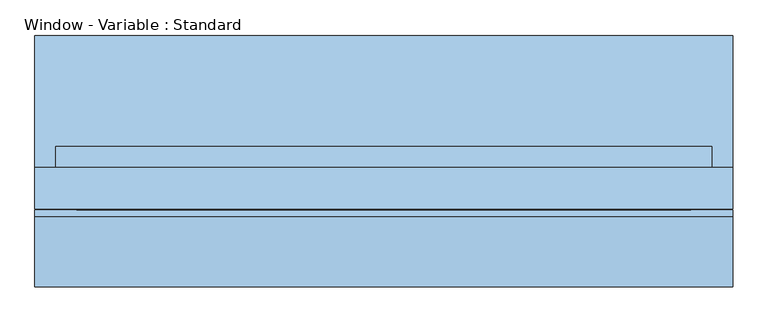
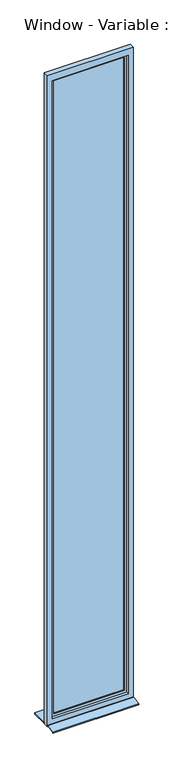
"""IFC4 building model written with IfcOpenShell, lengths in millimetres: window geometry, Window - Variable : Standard."""

from ifc_helpers import new_model, si_unit, frame, origin, place, context, project, spatial, polyline, outline, extrude, faceted_brep, source, transform, mapped, element, save


def window_variable_standard_9eb8f332(model_context):
    return source(origin(), model_context, "Body", "SolidModel", [
        extrude(outline(polyline([(9000.0, 500.0), (9000.0, -500.0), (1000.0, -500.0), (1000.0, 500.0), (9000.0, 500.0)]), holes=[polyline([(8920.0, 440.0), (1080.0, 440.0), (1080.0, -440.0), (8920.0, -440.0), (8920.0, 440.0)])]), frame((0.0, -70.0, 0.0), z_axis=(0.0, 1.0, 0.0), x_axis=(0.0, 0.0, 1.0)), (0.0, 0.0, 1.0), 60.0),
        faceted_brep([(470.0, -10.0, 8950.0), (470.0, -10.0, 1050.0), (470.0, 20.0, 1050.0), (470.0, 20.0, 8950.0), (-470.0, 20.0, 1050.0), (-470.0, 20.0, 8950.0), (410.0, 20.0, 1110.0), (410.0, 20.0, 8890.0), (-410.0, 20.0, 8890.0), (-410.0, 20.0, 1110.0), (-470.0, -10.0, 1050.0), (-470.0, -10.0, 8950.0), (440.0, -10.0, 8920.0), (440.0, -10.0, 1080.0), (-440.0, -10.0, 1080.0), (-440.0, -10.0, 8920.0), (440.0, -40.0, 8920.0), (440.0, -40.0, 1080.0), (-440.0, -40.0, 1080.0), (-440.0, -40.0, 8920.0), (410.0, -40.0, 8890.0), (410.0, -40.0, 1110.0), (-410.0, -40.0, 1110.0), (-410.0, -40.0, 8890.0)], [[[0, 1, 2, 3]], [[3, 2, 4, 5], [6, 7, 8, 9]], [[1, 10, 4, 2]], [[1, 0, 11, 10], [12, 13, 14, 15]], [[16, 17, 13, 12]], [[17, 18, 14, 13]], [[17, 16, 19, 18], [20, 21, 22, 23]], [[7, 6, 21, 20]], [[6, 9, 22, 21]], [[10, 11, 5, 4]], [[18, 19, 15, 14]], [[9, 8, 23, 22]], [[11, 0, 3, 5]], [[19, 16, 12, 15]], [[8, 7, 20, 23]]]),
        extrude(outline(polyline([(-500.0, 180.0), (500.0, 180.0), (500.0, -10.0), (-500.0, -10.0), (-500.0, 180.0)])), frame((0.0, 0.0, 1005.0), z_axis=(0.0, 0.0, 1.0), x_axis=(1.0, 0.0, 0.0)), (0.0, 0.0, 1.0), 15.0),
        extrude(outline(polyline([(-80.0221543, 1020.0), (-70.0, 1020.0), (-70.0, 1018.0), (-79.8240723, 1018.0), (-178.0, 998.3604634), (-178.0, 990.0), (-180.0, 990.0), (-180.0, 1000.0), (-80.0221543, 1020.0)])), frame((-500.0, 0.0, 0.0), z_axis=(1.0, 0.0, 0.0), x_axis=(0.0, 1.0, 0.0)), (0.0, 0.0, 1.0), 1000.0),
        extrude(outline(polyline([(410.0, 5.0), (410.0, -25.0), (-410.0, -25.0), (-410.0, 5.0), (410.0, 5.0)])), frame((0.0, 0.0, 1110.0), z_axis=(0.0, 0.0, 1.0), x_axis=(1.0, 0.0, 0.0)), (0.0, 0.0, 1.0), 7780.0),
    ])


if __name__ == "__main__":
    model = new_model("IFC4")
    model_context = context("Model", 3, world=origin())
    ifc_project = project(units=[si_unit("LENGTHUNIT", "METRE", prefix="MILLI")], contexts=[model_context])
    site = spatial("IfcSite", under=ifc_project)
    building = spatial("IfcBuilding", under=site)
    placement = place(None, origin())
    window_variable_standard_shape = window_variable_standard_9eb8f332(model_context)
    element("IfcWindow", 1, ObjectType="Window - Variable : Standard", at=placement, inside=building, context=model_context, shape_type="MappedRepresentation", body=[
        mapped(window_variable_standard_shape, transform((0.0, 0.0, 0.0), x_axis=(1.0, 0.0, 0.0), y_axis=(0.0, 1.0, 0.0), z_axis=(0.0, 0.0, 1.0))),
    ])
    save(model, "model.ifc")

# Revit data of these elements
# Type "Window - Variable : Standard"
#   Type Mark = "19"
#   Operation = "SinglePanel"
#   Keynote = "16.05.01"
#   Analytic Construction = "<None>"
#   Rough Width [instance default] = 1.010 m
#   Rough Height [instance default] = 1.010 m
#   Frame Depth = 0.060 m
#   Frame Height Bottom = 0.080 m
#   Frame Height Top = 0.080 m
#   Frame Width = 0.060 m
#   Height [instance default] = 1.010 m
#   Window Inset = 0.060 m
#   Window Width = 0.060 m
#   Instalation Depth [instance default] = 0.080 m
#   Width [instance default] = 1.010 m
#   Folding Wing [instance default] = no
#   Oppening Direction Vertical [instance default] = yes
#   Oppening Direction Visibility [instance default] = no
#   Casement [instance default] = yes
#   Frame [instance default] = none
#   Glas [instance default] = none
#   Window [instance default] = none
#   Windowsill Inside [instance default] = none
#   Windowsill Outside [instance default] = none
#   Wall Closure = (empty or 0)
#   Assembly Code = ""
# Element 1 (IfcWindow, "Window - Variable : Standard")
#   Rough Width = 1.000 m
#   Rough Height = 8.000 m
#   Height = 8.000 m
#   Width = 1.000 m
#   Materials on its faces: "Plastic - White", "Metal _ Aluminium", "Wood - Birch", "Glass"
# Materials
#   "Plastic - White": class "Kunststoff", colour RGB 249 249 249, transparency 0
#   "Metal _ Aluminium": class "Metall", colour RGB 247 247 247, transparency 0
#   "Wood - Birch": class "Holz", colour RGB 213 164 103, transparency 0
#   "Glass": class "Glass", colour RGB 0 128 192, transparency 0.9
